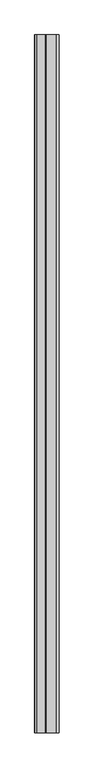
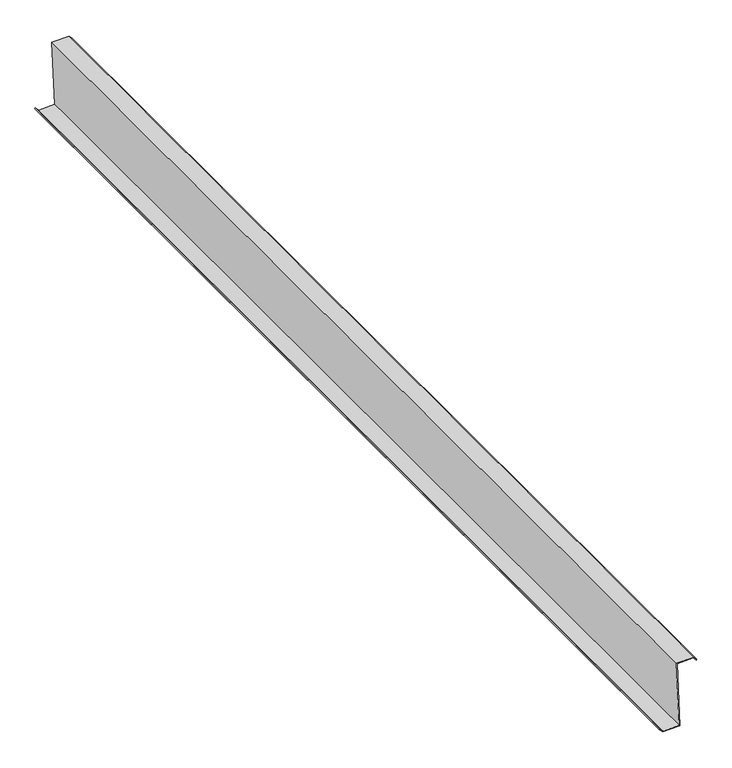
"""IFC4 building model written with IfcOpenShell, lengths in millimetres: proxy geometry, Generic Models 7:Generic Models 1:337419:Generic Models 1:337419 : Generic Models 7:Generic Models 1:337419:4 : Generic Models 7:Generic Models 1:337419:Generic Models 1:337419 : Generic Models 7:Generic Models 1:337419:301336."""

from ifc_helpers import new_model, si_unit, frame, origin, place, context, project, spatial, polyline, outline, extrude, source, transform, mapped, element, save


def generic_models_8eab5329(model_context):
    return source(origin(), model_context, "Body", "SweptSolid", [
        extrude(outline(polyline([(4107.8682634, 570868.3579207), (4358.8723474, 570857.8994172), (4361.4041288, 570918.6621711), (4348.110733, 570930.7947306), (4350.1630511, 570932.6828632), (4364.2337762, 570919.8408542), (4361.5324091, 570855.0080458), (4110.5283251, 570865.4665493), (4107.9965437, 570804.7037953), (4121.1104145, 570792.735084), (4119.0580965, 570790.8469514), (4105.1668964, 570803.5251122), (4107.8682634, 570868.3579207)])), frame((0.0, -578999.1038841, 0.0), z_axis=(0.0, 1.0, 0.0), x_axis=(0.0, 0.0, 1.0)), (0.0, 0.0, 1.0), 4094.7624605),
    ])


if __name__ == "__main__":
    model = new_model("IFC4")
    model_context = context("Model", 3, world=origin())
    ifc_project = project(units=[si_unit("LENGTHUNIT", "METRE", prefix="MILLI")], contexts=[model_context])
    site = spatial("IfcSite", under=ifc_project)
    building = spatial("IfcBuilding", under=site)
    placement = place(None, origin())
    generic_models_shape = generic_models_8eab5329(model_context)
    element("IfcBuildingElementProxy", 1, Name="Generic Models 7:Generic Models 1:337419:Generic Models 1:337419 : Generic Models 7:Generic Models 1:337419:4 : Generic Models 7:Generic Models 1:337419:Generic Models 1:337419 : Generic Models 7:Generic Models 1:337419:301336", ObjectType="Generic Models 7:Generic Models 1:337419:Generic Models 1:337419 : Generic Models 7:Generic Models 1:337419:4 : Generic Models 7:Generic Models 1:337419:Generic Models 1:337419 : Generic Models 7:Generic Models 1:337419:301336", at=placement, inside=building, context=model_context, shape_type="MappedRepresentation", body=[
        mapped(generic_models_shape, transform((0.0, 0.0, 0.0), x_axis=(1.0, 0.0, 0.0), y_axis=(0.0, 1.0, 0.0), z_axis=(0.0, 0.0, 1.0))),
    ])
    save(model, "model.ifc")

# Revit data of these elements
# Type "Generic Models 7:Generic Models 1:337419:Generic Models 1:337419 : Generic Models 7:Generic Models 1:337419:4 : Generic Models 7:Generic Models 1:337419:Generic Models 1:337419 : Generic Models 7:Generic Models 1:337419:301336"
#   NameOverride = "Generic Models 7:Generic Models 1:337419:Generic Models 1:337419 : Generic Models 7:Generic Models 1:337419:301336"
#   ObjectTypeOverride = "Generic Models 1:337419 : Generic Models 7:Generic Models 1:337419"
#   Reference = "Generic Models 1"
#   Tag = "301336"
# Element 1 (IfcBuildingElementProxy, "Generic Models 7:Generic Models 1:337419:Generic Models 1:337419 : Generic Models 7:Generic Models 1:337419:4 : Generic Models 7:Generic Models 1:337419:Generic Models 1:337419 : Generic Models 7:Generic Models 1:337419:301336")
#   Materials on its faces: "'ZEE' SECTION (8.0x3.5Z - SEE STRUCT. DWGS)"
# Materials
#   "'ZEE' SECTION (8.0x3.5Z - SEE STRUCT. DWGS)": class "Unassigned", colour RGB 210 209 208, transparency 0, Keynote = "M05121300.02", Cost = 0
